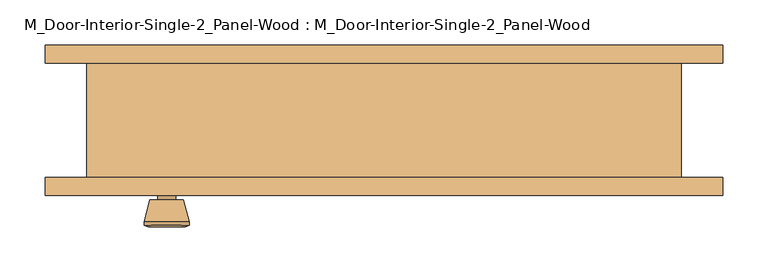
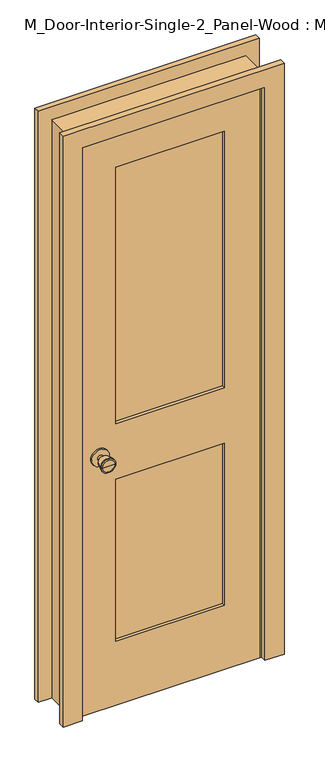
"""IFC4 building model written with IfcOpenShell, lengths in millimetres: door geometry, M_Door-Interior-Single-2_Panel-Wood : M_Door-Interior-Single-2_Panel-Wood."""

from ifc_helpers import new_model, si_unit, point, frame, frame_2d, origin, place, context, project, spatial, polyline, circle_curve, trimmed, segment, composite_curve, outline, extrude, faceted_brep, source, transform, mapped, element, save
from ifc_brep_helpers import plane_surface, cylinder_surface, revolved_surface, advanced_brep


def m_door_interior_single_2_panel_wood_m_door_interior_single_2_88952c05(model_context):
    return source(origin(), model_context, "Body", "SolidModel", [
        advanced_brep(
        [(-241.3, -19.325, 914.4), (-251.3, -19.325, 914.4), (-231.3, -19.325, 914.4), (-220.8241324, 29.675, 914.4), (-261.7758676, 29.675, 914.4), (-241.3, 29.675, 914.4), (-216.3, 27.8471319, 914.4), (-266.3, 27.8471319, 914.4), (-216.3, 24.3834537, 914.4), (-266.3, 24.3834537, 914.4), (-222.663764, -0.325, 914.4), (-259.936236, -0.325, 914.4), (-231.3, -0.325, 914.4), (-251.3, -0.325, 914.4)],
        [
            (0, 1),
            (1, 2, circle_curve(frame((-241.3, -19.325, 914.4), z_axis=(0.0, -1.0, 0.0), x_axis=(-1.0, 0.0, 0.0)), 10.0)),
            (2, 0),
            (2, 1, circle_curve(frame((-241.3, -19.325, 914.4), z_axis=(0.0, -1.0, 0.0), x_axis=(-1.0, 0.0, 0.0)), 10.0)),
            (3, 4, circle_curve(frame((-241.3, 29.675, 914.4), z_axis=(0.0, 1.0, 0.0), x_axis=(-1.0, 0.0, 0.0)), 20.4758676)),
            (4, 5),
            (5, 3),
            (4, 3, circle_curve(frame((-241.3, 29.675, 914.4), z_axis=(0.0, 1.0, 0.0), x_axis=(-1.0, 0.0, 0.0)), 20.4758676)),
            (6, 7, circle_curve(frame((-241.3, 27.8471319, 914.4), z_axis=(0.0, 1.0, 0.0), x_axis=(-1.0, 0.0, 0.0)), 25.0)),
            (7, 4),
            (3, 6),
            (7, 6, circle_curve(frame((-241.3, 27.8471319, 914.4), z_axis=(0.0, 1.0, 0.0), x_axis=(-1.0, 0.0, 0.0)), 25.0)),
            (8, 9, circle_curve(frame((-241.3, 24.3834537, 914.4), z_axis=(0.0, 1.0, 0.0), x_axis=(-1.0, 0.0, 0.0)), 25.0)),
            (9, 7),
            (6, 8),
            (9, 8, circle_curve(frame((-241.3, 24.3834537, 914.4), z_axis=(0.0, 1.0, 0.0), x_axis=(-1.0, 0.0, 0.0)), 25.0)),
            (10, 11, circle_curve(frame((-241.3, -0.325, 914.4), z_axis=(0.0, 1.0, 0.0), x_axis=(-1.0, 0.0, 0.0)), 18.636236)),
            (11, 9),
            (8, 10),
            (11, 10, circle_curve(frame((-241.3, -0.325, 914.4), z_axis=(0.0, 1.0, 0.0), x_axis=(-1.0, 0.0, 0.0)), 18.636236)),
            (12, 13, circle_curve(frame((-241.3, -0.325, 914.4), z_axis=(0.0, 1.0, 0.0), x_axis=(-1.0, 0.0, 0.0)), 10.0)),
            (13, 11),
            (10, 12),
            (13, 12, circle_curve(frame((-241.3, -0.325, 914.4), z_axis=(0.0, 1.0, 0.0), x_axis=(-1.0, 0.0, 0.0)), 10.0)),
            (1, 13),
            (12, 2),
        ],
        [
            plane_surface(frame((-241.3, -19.325, 914.4), z_axis=(0.0, -1.0, 0.0), x_axis=(-1.0, 0.0, 0.0))),
            plane_surface(frame((-241.3, 29.675, 914.4), z_axis=(0.0, 1.0, 0.0), x_axis=(-1.0, 0.0, 0.0))),
            revolved_surface(polyline([(-261.7758676, 29.675, 914.4), (-266.3, 27.8471319, 914.4)]), (-241.3, -19.325, 914.4), (0.0, -1.0, 0.0)),
            cylinder_surface(frame((-241.3, -19.325, 914.4), z_axis=(0.0, -1.0, 0.0), x_axis=(-1.0, 0.0, 0.0)), 25.0),
            revolved_surface(polyline([(-266.3, 24.3834537, 914.4), (-259.936236, -0.325, 914.4)]), (-241.3, -19.325, 914.4), (0.0, -1.0, 0.0)),
            plane_surface(frame((-241.3, -0.325, 914.4), z_axis=(0.0, -1.0, 0.0), x_axis=(-1.0, 0.0, 0.0))),
            cylinder_surface(frame((-241.3, -19.325, 914.4), z_axis=(0.0, -1.0, 0.0), x_axis=(-1.0, 0.0, 0.0)), 10.0),
        ],
        [
            (0, [[1, 2, 3]]),
            (0, [[-3, 4, -1]]),
            (1, [[5, 6, 7]]),
            (1, [[8, -7, -6]]),
            (2, [[9, 10, -5, 11]]),
            (2, [[12, -11, -8, -10]]),
            (3, [[13, 14, -9, 15]]),
            (3, [[16, -15, -12, -14]]),
            (4, [[17, 18, -13, 19]]),
            (4, [[20, -19, -16, -18]]),
            (5, [[21, 22, -17, 23]]),
            (5, [[24, -23, -20, -22]]),
            (6, [[-2, 25, -21, 26]]),
            (6, [[-4, -26, -24, -25]]),
        ],
    ),
        extrude(outline(composite_curve([segment(trimmed(circle_curve(frame_2d((914.4, -241.3)), 30.0), [point((914.4, -271.3))], [point((914.4, -211.3))], False, "CARTESIAN"), True, "CONTINUOUS"), segment(trimmed(circle_curve(frame_2d((914.4, -241.3)), 30.0), [point((914.4, -211.3))], [point((914.4, -271.3))], False, "CARTESIAN"), True, "CONTINUOUS")], self_intersect=False)), frame((0.0, -25.325, 0.0), z_axis=(0.0, 1.0, 0.0), x_axis=(0.0, 0.0, 1.0)), (0.0, 0.0, 1.0), 6.0),
        advanced_brep(
        [(-241.3, -66.325, 914.4), (-231.3, -66.325, 914.4), (-251.3, -66.325, 914.4), (-220.8241324, -115.325, 914.4), (-241.3, -115.325, 914.4), (-261.7758676, -115.325, 914.4), (-216.3, -113.4971319, 914.4), (-266.3, -113.4971319, 914.4), (-216.3, -110.0334537, 914.4), (-266.3, -110.0334537, 914.4), (-222.663764, -85.325, 914.4), (-259.936236, -85.325, 914.4), (-231.3, -85.325, 914.4), (-251.3, -85.325, 914.4)],
        [
            (0, 1),
            (1, 2, circle_curve(frame((-241.3, -66.325, 914.4), z_axis=(0.0, 1.0, 0.0), x_axis=(-1.0, 0.0, 0.0)), 10.0)),
            (2, 0),
            (2, 1, circle_curve(frame((-241.3, -66.325, 914.4), z_axis=(0.0, 1.0, 0.0), x_axis=(-1.0, 0.0, 0.0)), 10.0)),
            (3, 4),
            (4, 5),
            (5, 3, circle_curve(frame((-241.3, -115.325, 914.4), z_axis=(0.0, -1.0, 0.0), x_axis=(-1.0, 0.0, 0.0)), 20.4758676)),
            (3, 5, circle_curve(frame((-241.3, -115.325, 914.4), z_axis=(0.0, -1.0, 0.0), x_axis=(-1.0, 0.0, 0.0)), 20.4758676)),
            (6, 3),
            (5, 7),
            (7, 6, circle_curve(frame((-241.3, -113.4971319, 914.4), z_axis=(0.0, -1.0, 0.0), x_axis=(-1.0, 0.0, 0.0)), 25.0)),
            (6, 7, circle_curve(frame((-241.3, -113.4971319, 914.4), z_axis=(0.0, -1.0, 0.0), x_axis=(-1.0, 0.0, 0.0)), 25.0)),
            (8, 6),
            (7, 9),
            (9, 8, circle_curve(frame((-241.3, -110.0334537, 914.4), z_axis=(0.0, -1.0, 0.0), x_axis=(-1.0, 0.0, 0.0)), 25.0)),
            (8, 9, circle_curve(frame((-241.3, -110.0334537, 914.4), z_axis=(0.0, -1.0, 0.0), x_axis=(-1.0, 0.0, 0.0)), 25.0)),
            (10, 8),
            (9, 11),
            (11, 10, circle_curve(frame((-241.3, -85.325, 914.4), z_axis=(0.0, -1.0, 0.0), x_axis=(-1.0, 0.0, 0.0)), 18.636236)),
            (10, 11, circle_curve(frame((-241.3, -85.325, 914.4), z_axis=(0.0, -1.0, 0.0), x_axis=(-1.0, 0.0, 0.0)), 18.636236)),
            (12, 10),
            (11, 13),
            (13, 12, circle_curve(frame((-241.3, -85.325, 914.4), z_axis=(0.0, -1.0, 0.0), x_axis=(-1.0, 0.0, 0.0)), 10.0)),
            (12, 13, circle_curve(frame((-241.3, -85.325, 914.4), z_axis=(0.0, -1.0, 0.0), x_axis=(-1.0, 0.0, 0.0)), 10.0)),
            (1, 12),
            (13, 2),
        ],
        [
            plane_surface(frame((-241.3, -66.325, 914.4), z_axis=(0.0, 1.0, 0.0), x_axis=(-1.0, 0.0, 0.0))),
            plane_surface(frame((-241.3, -115.325, 914.4), z_axis=(0.0, -1.0, 0.0), x_axis=(-1.0, 0.0, 0.0))),
            revolved_surface(polyline([(-261.7758676, -115.325, 914.4), (-266.3, -113.4971319, 914.4)]), (-241.3, -66.325, 914.4), (0.0, 1.0, 0.0)),
            cylinder_surface(frame((-241.3, -66.325, 914.4), z_axis=(0.0, 1.0, 0.0), x_axis=(-1.0, 0.0, 0.0)), 25.0),
            revolved_surface(polyline([(-266.3, -110.0334537, 914.4), (-259.936236, -85.325, 914.4)]), (-241.3, -66.325, 914.4), (0.0, 1.0, 0.0)),
            plane_surface(frame((-241.3, -85.325, 914.4), z_axis=(0.0, 1.0, 0.0), x_axis=(-1.0, 0.0, 0.0))),
            cylinder_surface(frame((-241.3, -66.325, 914.4), z_axis=(0.0, 1.0, 0.0), x_axis=(-1.0, 0.0, 0.0)), 10.0),
        ],
        [
            (0, [[1, 2, 3]]),
            (0, [[-3, 4, -1]]),
            (1, [[5, 6, 7]]),
            (1, [[-6, -5, 8]]),
            (2, [[9, -7, 10, 11]]),
            (2, [[-10, -8, -9, 12]]),
            (3, [[13, -11, 14, 15]]),
            (3, [[-14, -12, -13, 16]]),
            (4, [[17, -15, 18, 19]]),
            (4, [[-18, -16, -17, 20]]),
            (5, [[21, -19, 22, 23]]),
            (5, [[-22, -20, -21, 24]]),
            (6, [[25, -23, 26, -2]]),
            (6, [[-26, -24, -25, -4]]),
        ],
    ),
        extrude(outline(composite_curve([segment(trimmed(circle_curve(frame_2d((914.4, -241.3)), 30.0), [point((914.4, -271.3))], [point((914.4, -211.3))], False, "CARTESIAN"), True, "CONTINUOUS"), segment(trimmed(circle_curve(frame_2d((914.4, -241.3)), 30.0), [point((914.4, -211.3))], [point((914.4, -271.3))], False, "CARTESIAN"), True, "CONTINUOUS")], self_intersect=False)), frame((0.0, -66.325, 0.0), z_axis=(0.0, 1.0, 0.0), x_axis=(0.0, 0.0, 1.0)), (0.0, 0.0, 1.0), 6.0),
        extrude(outline(polyline([(184.8, -36.9916667), (184.8, -48.6583333), (-184.8, -48.6583333), (-184.8, -36.9916667), (184.8, -36.9916667)])), frame((0.0, 0.0, 1014.4), z_axis=(0.0, 0.0, 1.0), x_axis=(1.0, 0.0, 0.0)), (0.0, 0.0, 1.0), 923.0),
        extrude(outline(polyline([(184.8, -36.9916667), (184.8, -48.6583333), (-184.8, -48.6583333), (-184.8, -36.9916667), (184.8, -36.9916667)])), frame((0.0, 0.0, 230.0), z_axis=(0.0, 0.0, 1.0), x_axis=(1.0, 0.0, 0.0)), (0.0, 0.0, 1.0), 584.4),
        extrude(outline(polyline([(2057.4, -304.8), (0.0, -304.8), (0.0, 304.8), (2057.4, 304.8), (2057.4, -304.8)]), holes=[polyline([(1937.4, -184.8), (1937.4, 184.8), (1014.4, 184.8), (1014.4, -184.8), (1937.4, -184.8)]), polyline([(814.4, -184.8), (814.4, 184.8), (230.0, 184.8), (230.0, -184.8), (814.4, -184.8)])]), frame((0.0, -60.325, 0.0), z_axis=(0.0, 1.0, 0.0), x_axis=(0.0, 0.0, 1.0)), (0.0, 0.0, 1.0), 35.0),
        faceted_brep([(329.8, -60.325, 0.0), (304.8, -60.325, 0.0), (304.8, -25.325, 0.0), (292.1, -25.325, 0.0), (292.1, 9.6, 0.0), (304.8, 9.6, 0.0), (304.8, 66.675, 0.0), (329.8, 66.675, 0.0), (329.8, 66.675, 2082.4), (329.8, -60.325, 2082.4), (304.8, 66.675, 2057.4), (-304.8, 66.675, 2057.4), (-304.8, 66.675, 0.0), (-329.8, 66.675, 0.0), (-329.8, 66.675, 2082.4), (304.8, 9.6, 2057.4), (292.1, 9.6, 2044.7), (-292.1, 9.6, 2044.7), (-292.1, 9.6, 0.0), (-304.8, 9.6, 0.0), (-304.8, 9.6, 2057.4), (292.1, -25.325, 2044.7), (304.8, -25.325, 2057.4), (-304.8, -25.325, 2057.4), (-304.8, -25.325, 0.0), (-292.1, -25.325, 0.0), (-292.1, -25.325, 2044.7), (304.8, -60.325, 2057.4), (-329.8, -60.325, 2082.4), (-329.8, -60.325, 0.0), (-304.8, -60.325, 0.0), (-304.8, -60.325, 2057.4)], [[[0, 1, 2, 3, 4, 5, 6, 7]], [[7, 8, 9, 0]], [[6, 10, 11, 12, 13, 14, 8, 7]], [[5, 15, 10, 6]], [[4, 16, 17, 18, 19, 20, 15, 5]], [[3, 21, 16, 4]], [[2, 22, 23, 24, 25, 26, 21, 3]], [[1, 27, 22, 2]], [[0, 9, 28, 29, 30, 31, 27, 1]], [[8, 14, 28, 9]], [[15, 20, 11, 10]], [[21, 26, 17, 16]], [[27, 31, 23, 22]], [[29, 13, 12, 19, 18, 25, 24, 30]], [[14, 13, 29, 28]], [[20, 19, 12, 11]], [[26, 25, 18, 17]], [[31, 30, 24, 23]]]),
        extrude(outline(polyline([(0.0, 376.15), (2128.75, 376.15), (2128.75, -376.15), (0.0, -376.15), (0.0, -311.15), (2063.75, -311.15), (2063.75, 311.15), (0.0, 311.15), (0.0, 376.15)])), frame((0.0, 66.675, 0.0), z_axis=(0.0, 1.0, 0.0), x_axis=(0.0, 0.0, 1.0)), (0.0, 0.0, 1.0), 20.0),
        extrude(outline(polyline([(0.0, 376.15), (2128.75, 376.15), (2128.75, -376.15), (0.0, -376.15), (0.0, -311.15), (2063.75, -311.15), (2063.75, 311.15), (0.0, 311.15), (0.0, 376.15)])), frame((0.0, -80.325, 0.0), z_axis=(0.0, 1.0, 0.0), x_axis=(0.0, 0.0, 1.0)), (0.0, 0.0, 1.0), 20.0),
    ])


if __name__ == "__main__":
    model = new_model("IFC4")
    model_context = context("Model", 3, world=origin())
    ifc_project = project(units=[si_unit("LENGTHUNIT", "METRE", prefix="MILLI")], contexts=[model_context])
    site = spatial("IfcSite", under=ifc_project)
    building = spatial("IfcBuilding", under=site)
    placement = place(None, origin())
    m_door_interior_single_2_panel_wood_m_door_interior_single_2_shape = m_door_interior_single_2_panel_wood_m_door_interior_single_2_88952c05(model_context)
    element("IfcDoor", 1, ObjectType="M_Door-Interior-Single-2_Panel-Wood : M_Door-Interior-Single-2_Panel-Wood", at=placement, inside=building, context=model_context, shape_type="MappedRepresentation", body=[
        mapped(m_door_interior_single_2_panel_wood_m_door_interior_single_2_shape, transform((0.0, 0.0, 0.0), x_axis=(1.0, 0.0, 0.0), y_axis=(0.0, 1.0, 0.0), z_axis=(0.0, 0.0, 1.0))),
    ])
    save(model, "model.ifc")

# Revit data of these elements
# Type "M_Door-Interior-Single-2_Panel-Wood : M_Door-Interior-Single-2_Panel-Wood"
#   Type Mark = "i"
#   Assembly Code = "C1020300"
#   Analytic Construction = "Wooden"
#   Top Rail = 0' - 4.72441"
#   Thickness = 0' - 1.37795"
#   Thermal Resistance (R) = 0.455703 (m²·K)/W
#   Swing Angle [instance default] = 90.00°
#   Stiles = 0' - 4.72441"
#   Rough Width = 2' - 1.9685"
#   Rough Height = 6' - 9.98425"
#   Lock Rail = 0' - 7.87402"
#   Height = 6' - 9"
#   Width = 2' - 0"
#   Heat Transfer Coefficient (U) = 2.19465 W/(m²·K)
#   Bottom Rail = 0' - 9.05512"
#   Trim Material = Cherry
#   Panel Material = Cherry
#   Frame Material = Cherry
#   Door Handle Material = Aluminum
#   Visual Light Transmittance = 0
#   Solar Heat Gain Coefficient = 0
#   Wall Closure = (empty or 0)
#   Function = (empty or 0)
# Element 1 (IfcDoor, "M_Door-Interior-Single-2_Panel-Wood : M_Door-Interior-Single-2_Panel-Wood")
#   Materials on its faces: "Cherry", "Aluminum"
# Materials
#   "Cherry": class "Wood", colour RGB 154 107 61, transparency 0, Description = "Prunus Serotina", Cost = 0
#   "Aluminum": class "Metal", colour RGB 244 244 244, transparency 0, Description = "Aluminum 6061", Cost = 0
